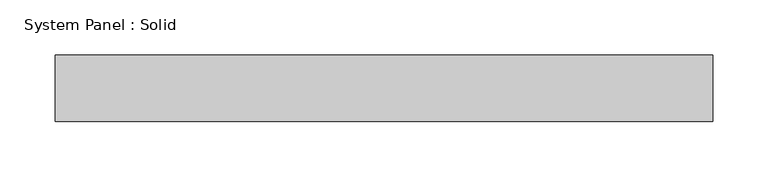
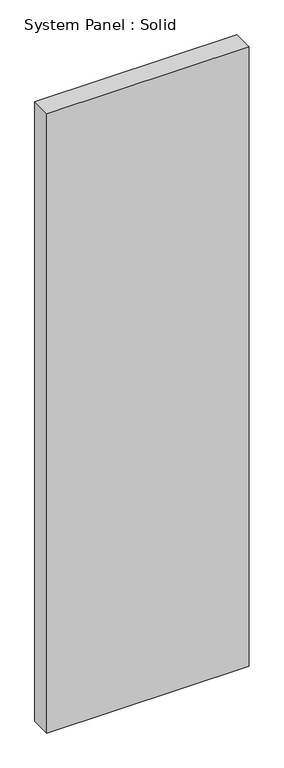
"""IFC4 building model written with IfcOpenShell, lengths in millimetres: plate geometry, System Panel : Solid."""

from ifc_helpers import new_model, si_unit, origin, origin_with_axes, place, context, project, spatial, polyline, outline, extrude, source, transform, mapped, element, save


def system_panel_solid_50642cbc(model_context):
    return source(origin(), model_context, "Body", "SweptSolid", [
        extrude(outline(polyline([(297.5, -10.5), (-297.5, -10.5), (-297.5, 49.5), (297.5, 49.5), (297.5, -10.5)])), origin_with_axes(), (0.0, 0.0, 1.0), 1925.0),
    ])


if __name__ == "__main__":
    model = new_model("IFC4")
    model_context = context("Model", 3, world=origin())
    ifc_project = project(units=[si_unit("LENGTHUNIT", "METRE", prefix="MILLI")], contexts=[model_context])
    site = spatial("IfcSite", under=ifc_project)
    building = spatial("IfcBuilding", under=site)
    placement = place(None, origin())
    system_panel_solid_shape = system_panel_solid_50642cbc(model_context)
    element("IfcPlate", 1, ObjectType="System Panel : Solid", at=placement, inside=building, context=model_context, shape_type="MappedRepresentation", body=[
        mapped(system_panel_solid_shape, transform((0.0, 0.0, 0.0), x_axis=(1.0, 0.0, 0.0), y_axis=(0.0, 1.0, 0.0), z_axis=(0.0, 0.0, 1.0))),
    ])
    save(model, "model.ifc")

# Revit data of these elements
# Element 1 (IfcPlate, "System Panel : Solid")
#   Materials on its faces: "Default"
# Materials
#   "Default": class "Miscellaneous", colour RGB 127 127 127, transparency 0
